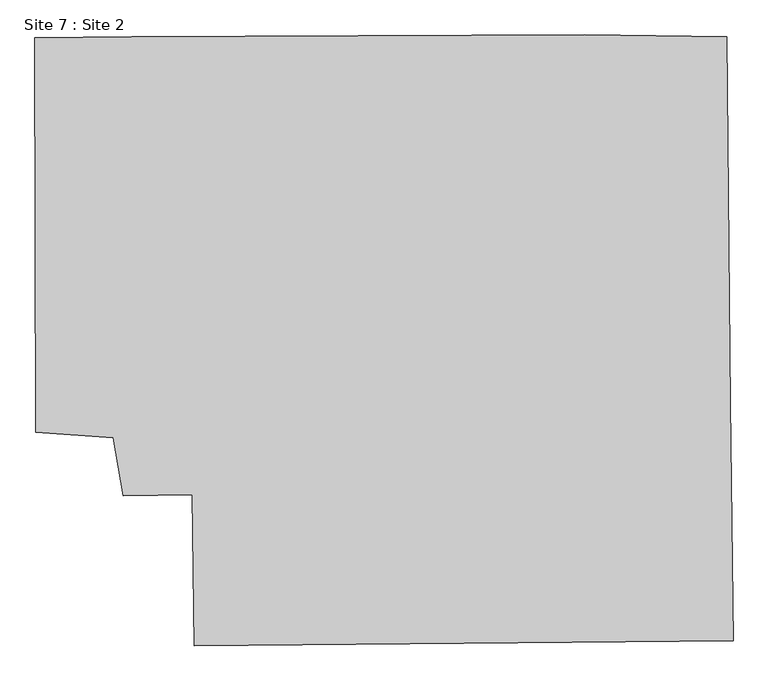
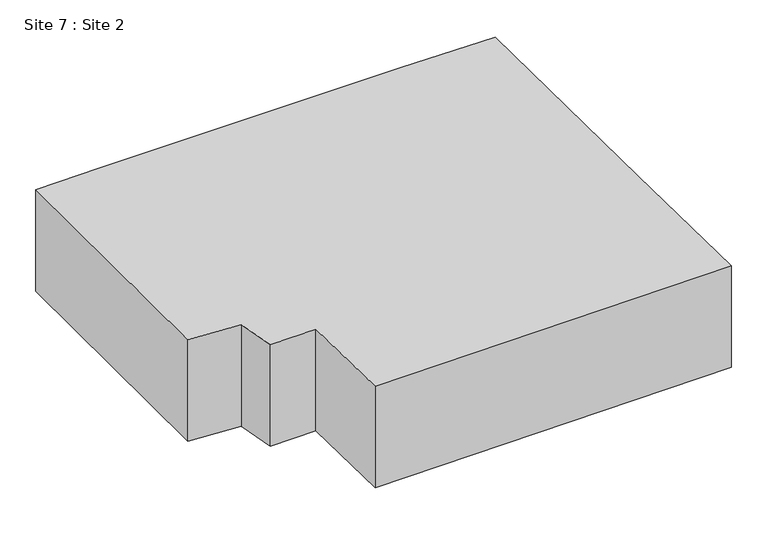
"""IFC4 building model written with IfcOpenShell, lengths in millimetres: geographic element geometry, Site 7 : Site 2."""

import ifcopenshell
import ifcopenshell.guid

model = None  # the IFC model being written
_history = None  # IfcOwnerHistory: only IFC2X3 demands one
_inside = {}  # id of a spatial element -> (the spatial element, [elements in it])
_under = {}  # id of a project, library or spatial element -> (it, [spatial elements below it])
_declared = {}  # id of a project -> (the project, [libraries it declares])
_typed = {}  # id of a type object -> (the type object, [elements of that type])
_made_of = {}  # id of a material, layer set ... -> (it, [elements and type objects made of it])


def new_model(schema):
    """Start an empty IFC model of exactly this schema.

    Asked for "IFC4X3", IfcOpenShell would pick the latest addendum, in which some entities
    have other attributes; the version numbers below select the first issue.
    IFC2X3 requires an IfcOwnerHistory on every rooted entity: one is made here for all.
    """
    global model, _history
    if schema == "IFC4X3":
        model = ifcopenshell.file(schema_version=(4, 3, 0, 0))
    else:
        model = ifcopenshell.file(schema=schema)
    _inside.clear()
    _under.clear()
    _declared.clear()
    _typed.clear()
    _made_of.clear()
    _history = None
    if model.schema == "IFC2X3":
        org = make("IfcOrganization", Name="unknown")
        user = make(
            "IfcPersonAndOrganization",
            ThePerson=make("IfcPerson", FamilyName="unknown"),
            TheOrganization=org,
        )
        app = make(
            "IfcApplication",
            ApplicationDeveloper=org,
            Version="unknown",
            ApplicationFullName="unknown",
            ApplicationIdentifier="unknown",
        )
        _history = make(
            "IfcOwnerHistory",
            OwningUser=user,
            OwningApplication=app,
            ChangeAction="ADDED",
            CreationDate=0,
        )
    return model


def make(cls, **values):
    """One entity of the class cls with the attributes given. An attribute that is None is left unset."""
    return model.create_entity(
        cls, **{name: value for name, value in values.items() if value is not None}
    )


def rooted(cls, **values):
    """An entity with a GlobalId (a new one), such as an element, a storey or a relation."""
    return make(cls, GlobalId=ifcopenshell.guid.new(), OwnerHistory=_history, **values)


def si_unit(unit_type, name, prefix=None):
    """IfcSIUnit, for example si_unit("LENGTHUNIT", "METRE", prefix="MILLI")."""
    return make("IfcSIUnit", UnitType=unit_type, Prefix=prefix, Name=name)


def assignment(units):
    """IfcUnitAssignment: the units of a project."""
    return None if units is None else make("IfcUnitAssignment", Units=units)


def point(xyz):
    """IfcCartesianPoint."""
    return None if xyz is None else make("IfcCartesianPoint", Coordinates=xyz)


def direction(xyz):
    """IfcDirection."""
    return None if xyz is None else make("IfcDirection", DirectionRatios=xyz)


def frame(location, z_axis=None, x_axis=None):
    """IfcAxis2Placement3D, a coordinate frame: its origin and axes. An axis left out is left unset."""
    return make(
        "IfcAxis2Placement3D",
        Location=point(location),
        Axis=direction(z_axis),
        RefDirection=direction(x_axis),
    )


def origin():
    """The frame at (0, 0, 0) with its axes left unset."""
    return frame((0.0, 0.0, 0.0))


def place(relative_to, where):
    """IfcLocalPlacement: puts the frame where relative to a parent placement (None: the world)."""
    return make(
        "IfcLocalPlacement", PlacementRelTo=relative_to, RelativePlacement=where
    )


def context(
    kind, dimensions, precision=None, world=None, true_north=None, identifier=None
):
    """IfcGeometricRepresentationContext, for example the 3D "Model" context."""
    return make(
        "IfcGeometricRepresentationContext",
        ContextIdentifier=identifier,
        ContextType=kind,
        CoordinateSpaceDimension=dimensions,
        Precision=precision,
        WorldCoordinateSystem=world,
        TrueNorth=true_north,
    )


def project(units=None, contexts=None):
    """IfcProject with its units and contexts."""
    return rooted(
        "IfcProject",
        Name="project",
        RepresentationContexts=contexts,
        UnitsInContext=assignment(units),
    )


def spatial(cls, under=None, at=None, **own):
    """A site, building, storey or space (cls), placed at a placement, below another one or the project."""
    s = rooted(cls, ObjectPlacement=at, **own)
    if under is not None:
        _under.setdefault(under.id(), (under, []))[1].append(s)
    return s


def polyline(points):
    """IfcPolyline through the points."""
    return make("IfcPolyline", Points=[point(p) for p in points])


def outline(outer, holes=None, kind="AREA"):
    """IfcArbitraryClosedProfileDef: a profile drawn as a closed curve; with holes, ...WithVoids."""
    if holes is None:
        return make("IfcArbitraryClosedProfileDef", ProfileType=kind, OuterCurve=outer)
    return make(
        "IfcArbitraryProfileDefWithVoids",
        ProfileType=kind,
        OuterCurve=outer,
        InnerCurves=holes,
    )


def extrude(swept, where, along, depth):
    """IfcExtrudedAreaSolid: the profile swept, set in the frame where, extruded along a direction by depth."""
    return make(
        "IfcExtrudedAreaSolid",
        SweptArea=swept,
        Position=where,
        ExtrudedDirection=direction(along),
        Depth=depth,
    )


def shape(context_of_items, identifier, shape_type, items):
    """IfcShapeRepresentation: the items that make up one representation, for example the "Body"."""
    return make(
        "IfcShapeRepresentation",
        ContextOfItems=context_of_items,
        RepresentationIdentifier=identifier,
        RepresentationType=shape_type,
        Items=items,
    )


def source(mapping_origin, context_of_items, identifier, shape_type, items):
    """IfcRepresentationMap: a shape defined once, which mapped items show again and again."""
    return make(
        "IfcRepresentationMap",
        MappingOrigin=mapping_origin,
        MappedRepresentation=shape(context_of_items, identifier, shape_type, items),
    )


def transform(
    local_origin,
    x_axis=None,
    y_axis=None,
    z_axis=None,
    scale=None,
    scale2=None,
    scale3=None,
    uniform=True,
):
    """IfcCartesianTransformationOperator3D, or its non-uniform kind. x_axis, y_axis, z_axis: its Axis1, 2, 3."""
    if uniform:
        return make(
            "IfcCartesianTransformationOperator3D",
            Axis1=direction(x_axis),
            Axis2=direction(y_axis),
            LocalOrigin=point(local_origin),
            Scale=scale,
            Axis3=direction(z_axis),
        )
    return make(
        "IfcCartesianTransformationOperator3DnonUniform",
        Axis1=direction(x_axis),
        Axis2=direction(y_axis),
        LocalOrigin=point(local_origin),
        Scale=scale,
        Axis3=direction(z_axis),
        Scale2=scale2,
        Scale3=scale3,
    )


def mapped(mapping_source, mapping_target):
    """IfcMappedItem: shows the shape of a source again, moved by a transform."""
    return make(
        "IfcMappedItem", MappingSource=mapping_source, MappingTarget=mapping_target
    )


def made_of(thing, what):
    """Note that an element or type object is made of a material, layer set ...; save() writes the relation."""
    if what is not None:
        _made_of.setdefault(what.id(), (what, []))[1].append(thing)
    return thing


def element(
    cls,
    number,
    at=None,
    inside=None,
    cuts=None,
    type_object=None,
    material=None,
    context=None,
    identifier="Body",
    shape_type=None,
    held_by="IfcProductDefinitionShape",
    body=None,
    shapes=None,
    **own,
):
    """One element of the class cls, such as IfcWall. Its Tag is "e" and its number.

    at: its placement. inside: the storey or other place that contains it. cuts: it is an
    opening in that element (IfcRelVoidsElement). A single representation is given by context,
    identifier, shape_type and body (its items); several are given by shapes. held_by: the class
    of the entity that holds the representations. save() writes the other relations.
    """
    e = rooted(cls, Tag="e%d" % number, ObjectPlacement=at, **own)
    if body is not None:
        shapes = [shape(context, identifier, shape_type, body)]
    if shapes is not None:
        e.Representation = make(held_by, Representations=shapes)
    if inside is not None:
        _inside.setdefault(inside.id(), (inside, []))[1].append(e)
    if cuts is not None:
        rooted(
            "IfcRelVoidsElement", RelatingBuildingElement=cuts, RelatedOpeningElement=e
        )
    if type_object is not None:
        _typed.setdefault(type_object.id(), (type_object, []))[1].append(e)
    return made_of(e, material)


def aggregate(whole, parts):
    """IfcRelAggregates: a whole, such as a stair, and the parts it consists of."""
    return rooted("IfcRelAggregates", RelatingObject=whole, RelatedObjects=parts)


def save(model, path):
    """Write the relations noted so far, then the file.

    IfcRelAggregates (storeys below a building ...), IfcRelContainedInSpatialStructure (elements
    in a storey), IfcRelDefinesByType, IfcRelAssociatesMaterial and IfcRelDeclares: one each for
    every whole, place, type object, material and project.
    """
    for whole, parts in _under.values():
        aggregate(whole, parts)
    for where, things in _inside.values():
        rooted(
            "IfcRelContainedInSpatialStructure",
            RelatedElements=things,
            RelatingStructure=where,
        )
    for kind, things in _typed.values():
        rooted("IfcRelDefinesByType", RelatedObjects=things, RelatingType=kind)
    for what, things in _made_of.values():
        rooted("IfcRelAssociatesMaterial", RelatedObjects=things, RelatingMaterial=what)
    for by, libraries in _declared.values():
        rooted("IfcRelDeclares", RelatingContext=by, RelatedDefinitions=libraries)
    model.write(path)


def site_7_site_2_ff44412e(model_context):
    return source(origin(), model_context, "Body", "SweptSolid", [
        extrude(outline(polyline([(-25965.0741058, 21462.89147), (-25822.1944366, 10283.8077133), (-51228.3606592, 10042.2224173), (-51328.5182912, 17156.3070396), (-54580.8499882, 17101.8159228), (-55049.0577043, 19852.0270273), (-58703.3306033, 20108.226609), (-58738.7748805, 38703.1705401), (-54165.78092, 38738.5288976), (-32826.1320487, 38835.809938), (-26121.2378387, 38738.6744849), (-25965.0741058, 21462.89147)])), frame((0.0, 0.0, 266395.2), z_axis=(0.0, 0.0, 1.0), x_axis=(1.0, 0.0, 0.0)), (0.0, 0.0, 1.0), 7620.0),
    ])


if __name__ == "__main__":
    model = new_model("IFC4")
    model_context = context("Model", 3, world=origin())
    ifc_project = project(units=[si_unit("LENGTHUNIT", "METRE", prefix="MILLI")], contexts=[model_context])
    site = spatial("IfcSite", under=ifc_project)
    building = spatial("IfcBuilding", under=site)
    placement = place(None, origin())
    site_7_site_2_shape = site_7_site_2_ff44412e(model_context)
    element("IfcGeographicElement", 1, ObjectType="Site 7 : Site 2", at=placement, inside=building, context=model_context, shape_type="MappedRepresentation", body=[
        mapped(site_7_site_2_shape, transform((0.0, 0.0, 0.0), x_axis=(1.0, 0.0, 0.0), y_axis=(0.0, 1.0, 0.0), z_axis=(0.0, 0.0, 1.0))),
    ])
    save(model, "model.ifc")

# Revit data of these elements
# Element 1 (IfcGeographicElement, "Site 7 : Site 2")
#   Materials on its faces: "EXISTING BUILDING"
# Materials
#   "EXISTING BUILDING": class "Generic", colour RGB 120 120 120, transparency 0, Cost = 0
